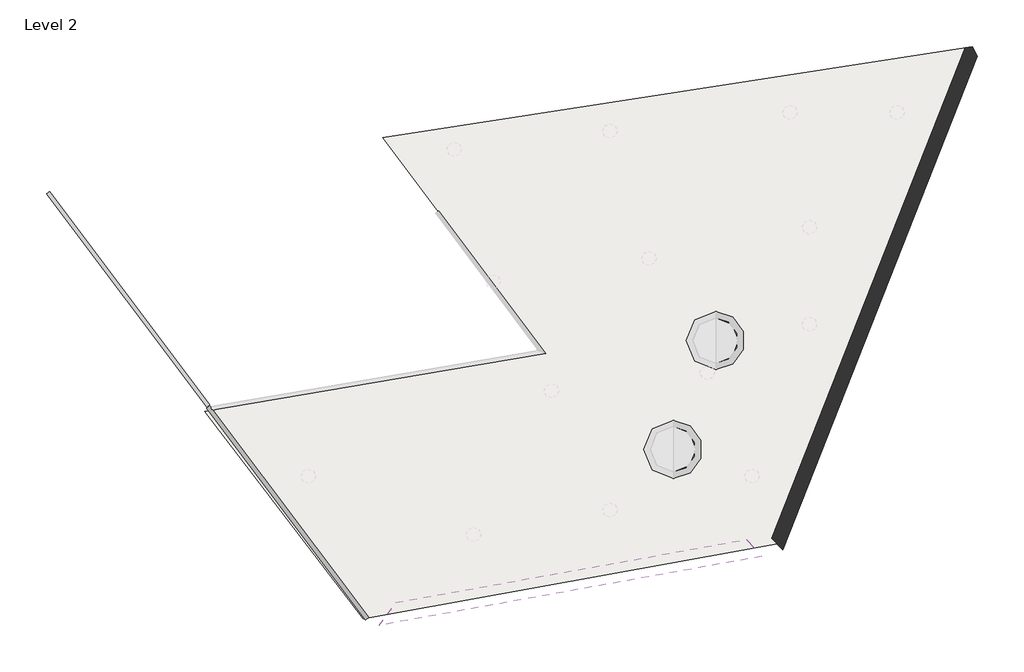
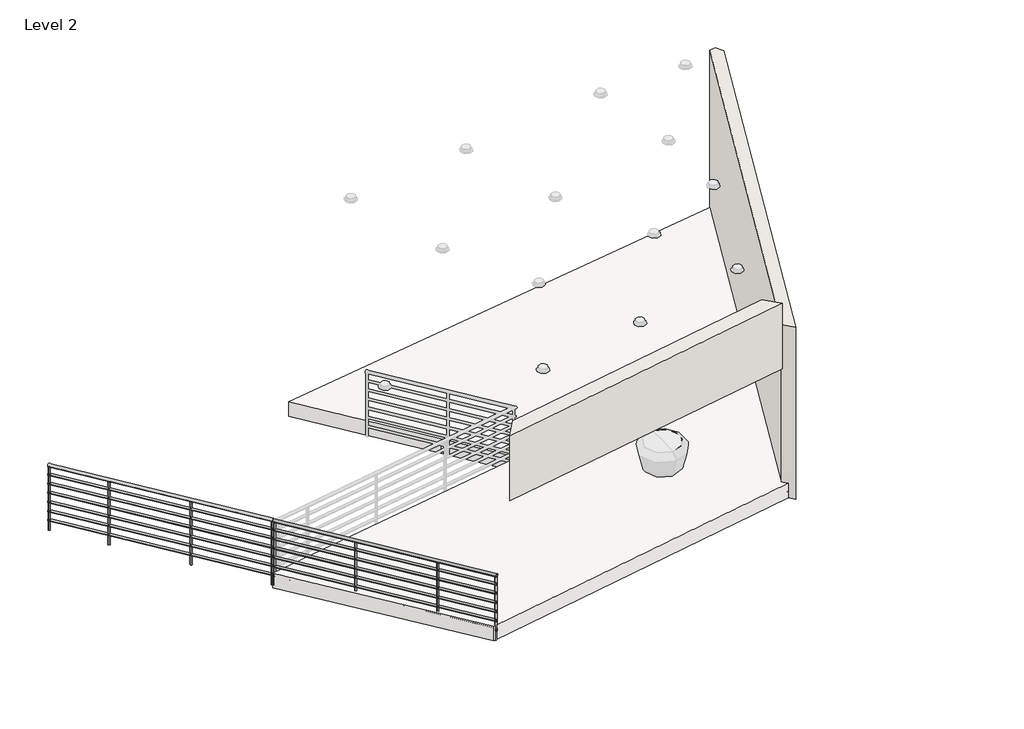
# One storey, part 1 of 2: 2 railings, 2 walls, 1 slab.
"""IFC4 building model written with IfcOpenShell, lengths in millimetres."""

from ifc_helpers import new_model, si_unit, point, frame, frame_2d, origin, place, context, project, spatial, polyline, circle_curve, trimmed, segment, composite_curve, outline, extrude, faceted_brep, element, save
from ifc_brep_helpers import plane_surface, revolved_surface, advanced_brep

model = new_model("IFC4")

# Units and contexts
model_context = context("Model", 3, world=origin())
ifc_project = project(units=[si_unit("LENGTHUNIT", "METRE", prefix="MILLI")], contexts=[model_context])

# Site, building, storey
site = spatial("IfcSite", under=ifc_project)
building = spatial("IfcBuilding", under=site)
storey = spatial("IfcBuildingStorey", under=building, Name="Level 2", Elevation=20000.0)

# Railings
placement = place(None, origin())
element("IfcRailing", 1, ObjectType="900mm Pipe", at=placement, inside=storey, context=model_context, shape_type="SweptSolid", body=[
    extrude(outline(composite_curve([segment(trimmed(circle_curve(frame_2d((0.0, 20.0)), 20.0), [point((-20.0, 20.0))], [point((20.0, 20.0))], False, "CARTESIAN"), True, "CONTINUOUS"), segment(trimmed(circle_curve(frame_2d((0.0, 20.0)), 20.0), [point((20.0, 20.0))], [point((-20.0, 20.0))], False, "CARTESIAN"), True, "CONTINUOUS")], self_intersect=False)), frame((80731.135292, 41327.5386845, 20900.0), z_axis=(-0.600141867985958, 0.7998935793531069, 0.0), x_axis=(0.7998935793531069, 0.600141867985958, 0.0)), (0.0, 0.0, 1.0), 2720.0),
    extrude(outline(composite_curve([segment(trimmed(circle_curve(frame_2d((0.0, 15.0)), 15.0), [point((15.0, 15.0))], [point((-15.0, 15.0))], False, "CARTESIAN"), True, "CONTINUOUS"), segment(trimmed(circle_curve(frame_2d((0.0, 15.0)), 15.0), [point((-15.0, 15.0))], [point((15.0, 15.0))], False, "CARTESIAN"), True, "CONTINUOUS")], self_intersect=False)), frame((80731.135292, 41327.5386845, 20775.0), z_axis=(-0.600141867985958, 0.7998935793531069, 0.0), x_axis=(0.7998935793531069, 0.600141867985958, 0.0)), (0.0, 0.0, 1.0), 2720.0),
    extrude(outline(composite_curve([segment(trimmed(circle_curve(frame_2d((0.0, 15.0)), 15.0), [point((15.0, 15.0))], [point((-15.0, 15.0))], False, "CARTESIAN"), True, "CONTINUOUS"), segment(trimmed(circle_curve(frame_2d((0.0, 15.0)), 15.0), [point((-15.0, 15.0))], [point((15.0, 15.0))], False, "CARTESIAN"), True, "CONTINUOUS")], self_intersect=False)), frame((80731.135292, 41327.5386845, 20650.0), z_axis=(-0.600141867985958, 0.7998935793531069, 0.0), x_axis=(0.7998935793531069, 0.600141867985958, 0.0)), (0.0, 0.0, 1.0), 2720.0),
    extrude(outline(composite_curve([segment(trimmed(circle_curve(frame_2d((0.0, 15.0)), 15.0), [point((15.0, 15.0))], [point((-15.0, 15.0))], False, "CARTESIAN"), True, "CONTINUOUS"), segment(trimmed(circle_curve(frame_2d((0.0, 15.0)), 15.0), [point((-15.0, 15.0))], [point((15.0, 15.0))], False, "CARTESIAN"), True, "CONTINUOUS")], self_intersect=False)), frame((80731.135292, 41327.5386845, 20525.0), z_axis=(-0.600141867985958, 0.7998935793531069, 0.0), x_axis=(0.7998935793531069, 0.600141867985958, 0.0)), (0.0, 0.0, 1.0), 2720.0),
    extrude(outline(composite_curve([segment(trimmed(circle_curve(frame_2d((0.0, 15.0)), 15.0), [point((15.0, 15.0))], [point((-15.0, 15.0))], False, "CARTESIAN"), True, "CONTINUOUS"), segment(trimmed(circle_curve(frame_2d((0.0, 15.0)), 15.0), [point((-15.0, 15.0))], [point((15.0, 15.0))], False, "CARTESIAN"), True, "CONTINUOUS")], self_intersect=False)), frame((80731.135292, 41327.5386845, 20400.0), z_axis=(-0.600141867985958, 0.7998935793531069, 0.0), x_axis=(0.7998935793531069, 0.600141867985958, 0.0)), (0.0, 0.0, 1.0), 2720.0),
    extrude(outline(composite_curve([segment(trimmed(circle_curve(frame_2d((0.0, 15.0)), 15.0), [point((15.0, 15.0))], [point((-15.0, 15.0))], False, "CARTESIAN"), True, "CONTINUOUS"), segment(trimmed(circle_curve(frame_2d((0.0, 15.0)), 15.0), [point((-15.0, 15.0))], [point((15.0, 15.0))], False, "CARTESIAN"), True, "CONTINUOUS")], self_intersect=False)), frame((80731.135292, 41327.5386845, 20275.0), z_axis=(-0.600141867985958, 0.7998935793531069, 0.0), x_axis=(0.7998935793531069, 0.600141867985958, 0.0)), (0.0, 0.0, 1.0), 2720.0),
    extrude(outline(composite_curve([segment(trimmed(circle_curve(frame_2d((0.0, 15.0)), 15.0), [point((15.0, 15.0))], [point((-15.0, 15.0))], False, "CARTESIAN"), True, "CONTINUOUS"), segment(trimmed(circle_curve(frame_2d((0.0, 15.0)), 15.0), [point((-15.0, 15.0))], [point((15.0, 15.0))], False, "CARTESIAN"), True, "CONTINUOUS")], self_intersect=False)), frame((80731.135292, 41327.5386845, 20150.0), z_axis=(-0.600141867985958, 0.7998935793531069, 0.0), x_axis=(0.7998935793531069, 0.600141867985958, 0.0)), (0.0, 0.0, 1.0), 2720.0),
    extrude(outline(composite_curve([segment(trimmed(circle_curve(frame_2d((80299.033147, 41903.4620616)), 12.5), [point((80309.0318168, 41910.963835))], [point((80289.0344773, 41895.9602883))], False, "CARTESIAN"), True, "CONTINUOUS"), segment(trimmed(circle_curve(frame_2d((80299.033147, 41903.4620616)), 12.5), [point((80289.0344773, 41895.9602883))], [point((80309.0318168, 41910.963835))], False, "CARTESIAN"), True, "CONTINUOUS")], self_intersect=False)), frame((0.0, 0.0, 20000.0), z_axis=(0.0, 0.0, 1.0), x_axis=(1.0, 0.0, 0.0)), (0.0, 0.0, 1.0), 860.0),
    extrude(outline(composite_curve([segment(trimmed(circle_curve(frame_2d((79698.8912791, 42703.355641)), 12.5), [point((79708.8899488, 42710.8574143))], [point((79688.8926093, 42695.8538676))], False, "CARTESIAN"), True, "CONTINUOUS"), segment(trimmed(circle_curve(frame_2d((79698.8912791, 42703.355641)), 12.5), [point((79688.8926093, 42695.8538676))], [point((79708.8899488, 42710.8574143))], False, "CARTESIAN"), True, "CONTINUOUS")], self_intersect=False)), frame((0.0, 0.0, 20000.0), z_axis=(0.0, 0.0, 1.0), x_axis=(1.0, 0.0, 0.0)), (0.0, 0.0, 1.0), 860.0),
    extrude(outline(composite_curve([segment(trimmed(circle_curve(frame_2d((80723.6335186, 41337.5373543)), 12.5), [point((80733.6321884, 41345.0391276))], [point((80713.6348489, 41330.0355809))], False, "CARTESIAN"), True, "CONTINUOUS"), segment(trimmed(circle_curve(frame_2d((80723.6335186, 41337.5373543)), 12.5), [point((80713.6348489, 41330.0355809))], [point((80733.6321884, 41345.0391276))], False, "CARTESIAN"), True, "CONTINUOUS")], self_intersect=False)), frame((0.0, 0.0, 20000.0), z_axis=(0.0, 0.0, 1.0), x_axis=(1.0, 0.0, 0.0)), (0.0, 0.0, 1.0), 860.0),
    extrude(outline(composite_curve([segment(trimmed(circle_curve(frame_2d((79106.2511844, 43493.2505506)), 12.5), [point((79116.2498542, 43500.752324))], [point((79096.2525147, 43485.7487773))], False, "CARTESIAN"), True, "CONTINUOUS"), segment(trimmed(circle_curve(frame_2d((79106.2511844, 43493.2505506)), 12.5), [point((79096.2525147, 43485.7487773))], [point((79116.2498542, 43500.752324))], False, "CARTESIAN"), True, "CONTINUOUS")], self_intersect=False)), frame((0.0, 0.0, 20000.0), z_axis=(0.0, 0.0, 1.0), x_axis=(1.0, 0.0, 0.0)), (0.0, 0.0, 1.0), 860.0),
])
element("IfcRailing", 2, ObjectType="900mm Pipe", at=placement, inside=storey, context=model_context, shape_type="SweptSolid", body=[
    extrude(outline(composite_curve([segment(trimmed(circle_curve(frame_2d((0.0, 20.0)), 20.0), [point((20.0, 20.0))], [point((-20.0, 20.0))], False, "CARTESIAN"), True, "CONTINUOUS"), segment(trimmed(circle_curve(frame_2d((0.0, 20.0)), 20.0), [point((-20.0, 20.0))], [point((20.0, 20.0))], False, "CARTESIAN"), True, "CONTINUOUS")], self_intersect=False)), frame((79098.1923254, 43514.614153, 20900.0), z_axis=(-0.6001418679860292, 0.7998935793530534, 0.0), x_axis=(0.7998935793530534, 0.6001418679860292, 0.0)), (0.0, 0.0, 1.0), 2740.0),
    extrude(outline(composite_curve([segment(trimmed(circle_curve(frame_2d((0.0, 15.0)), 15.0), [point((-15.0, 15.0))], [point((15.0000001, 15.0))], False, "CARTESIAN"), True, "CONTINUOUS"), segment(trimmed(circle_curve(frame_2d((0.0, 15.0)), 15.0), [point((15.0000001, 15.0))], [point((-15.0, 15.0))], False, "CARTESIAN"), True, "CONTINUOUS")], self_intersect=False)), frame((79098.1923254, 43514.614153, 20775.0), z_axis=(-0.6001418679860292, 0.7998935793530534, 0.0), x_axis=(0.7998935793530534, 0.6001418679860292, 0.0)), (0.0, 0.0, 1.0), 2740.0),
    extrude(outline(composite_curve([segment(trimmed(circle_curve(frame_2d((0.0, 15.0)), 15.0), [point((-15.0, 15.0))], [point((15.0000001, 15.0))], False, "CARTESIAN"), True, "CONTINUOUS"), segment(trimmed(circle_curve(frame_2d((0.0, 15.0)), 15.0), [point((15.0000001, 15.0))], [point((-15.0, 15.0))], False, "CARTESIAN"), True, "CONTINUOUS")], self_intersect=False)), frame((79098.1923254, 43514.614153, 20650.0), z_axis=(-0.6001418679860292, 0.7998935793530534, 0.0), x_axis=(0.7998935793530534, 0.6001418679860292, 0.0)), (0.0, 0.0, 1.0), 2740.0),
    extrude(outline(composite_curve([segment(trimmed(circle_curve(frame_2d((0.0, 15.0)), 15.0), [point((-15.0, 15.0))], [point((15.0000001, 15.0))], False, "CARTESIAN"), True, "CONTINUOUS"), segment(trimmed(circle_curve(frame_2d((0.0, 15.0)), 15.0), [point((15.0000001, 15.0))], [point((-15.0, 15.0))], False, "CARTESIAN"), True, "CONTINUOUS")], self_intersect=False)), frame((79098.1923254, 43514.614153, 20525.0), z_axis=(-0.6001418679860292, 0.7998935793530534, 0.0), x_axis=(0.7998935793530534, 0.6001418679860292, 0.0)), (0.0, 0.0, 1.0), 2740.0),
    extrude(outline(composite_curve([segment(trimmed(circle_curve(frame_2d((0.0, 15.0)), 15.0), [point((-15.0, 15.0))], [point((15.0000001, 15.0))], False, "CARTESIAN"), True, "CONTINUOUS"), segment(trimmed(circle_curve(frame_2d((0.0, 15.0)), 15.0), [point((15.0000001, 15.0))], [point((-15.0, 15.0))], False, "CARTESIAN"), True, "CONTINUOUS")], self_intersect=False)), frame((79098.1923254, 43514.614153, 20400.0), z_axis=(-0.6001418679860292, 0.7998935793530534, 0.0), x_axis=(0.7998935793530534, 0.6001418679860292, 0.0)), (0.0, 0.0, 1.0), 2740.0),
    extrude(outline(composite_curve([segment(trimmed(circle_curve(frame_2d((0.0, 15.0)), 15.0), [point((-15.0, 15.0))], [point((15.0000001, 15.0))], False, "CARTESIAN"), True, "CONTINUOUS"), segment(trimmed(circle_curve(frame_2d((0.0, 15.0)), 15.0), [point((15.0000001, 15.0))], [point((-15.0, 15.0))], False, "CARTESIAN"), True, "CONTINUOUS")], self_intersect=False)), frame((79098.1923254, 43514.614153, 20275.0), z_axis=(-0.6001418679860292, 0.7998935793530534, 0.0), x_axis=(0.7998935793530534, 0.6001418679860292, 0.0)), (0.0, 0.0, 1.0), 2740.0),
    extrude(outline(composite_curve([segment(trimmed(circle_curve(frame_2d((0.0, 15.0)), 15.0), [point((-15.0, 15.0))], [point((15.0000001, 15.0))], False, "CARTESIAN"), True, "CONTINUOUS"), segment(trimmed(circle_curve(frame_2d((0.0, 15.0)), 15.0), [point((15.0000001, 15.0))], [point((-15.0, 15.0))], False, "CARTESIAN"), True, "CONTINUOUS")], self_intersect=False)), frame((79098.1923254, 43514.614153, 20150.0), z_axis=(-0.6001418679860292, 0.7998935793530534, 0.0), x_axis=(0.7998935793530534, 0.6001418679860292, 0.0)), (0.0, 0.0, 1.0), 2740.0),
    extrude(outline(composite_curve([segment(trimmed(circle_curve(frame_2d((77897.9085894, 45114.4013117)), 12.5), [point((77887.9099197, 45106.8995384))], [point((77907.9072591, 45121.9030851))], False, "CARTESIAN"), True, "CONTINUOUS"), segment(trimmed(circle_curve(frame_2d((77897.9085894, 45114.4013117)), 12.5), [point((77907.9072591, 45121.9030851))], [point((77887.9099197, 45106.8995384))], False, "CARTESIAN"), True, "CONTINUOUS")], self_intersect=False)), frame((0.0, 0.0, 20000.0), z_axis=(0.0, 0.0, 1.0), x_axis=(1.0, 0.0, 0.0)), (0.0, 0.0, 1.0), 860.0),
    extrude(outline(composite_curve([segment(trimmed(circle_curve(frame_2d((78498.0504574, 44314.5077324)), 12.5), [point((78488.0517876, 44307.005959))], [point((78508.0491271, 44322.0095057))], False, "CARTESIAN"), True, "CONTINUOUS"), segment(trimmed(circle_curve(frame_2d((78498.0504574, 44314.5077324)), 12.5), [point((78508.0491271, 44322.0095057))], [point((78488.0517876, 44307.005959))], False, "CARTESIAN"), True, "CONTINUOUS")], self_intersect=False)), frame((0.0, 0.0, 20000.0), z_axis=(0.0, 0.0, 1.0), x_axis=(1.0, 0.0, 0.0)), (0.0, 0.0, 1.0), 860.0),
    extrude(outline(composite_curve([segment(trimmed(circle_curve(frame_2d((77461.3053804, 45696.3238907)), 12.5), [point((77451.3067107, 45688.8221174))], [point((77471.3040502, 45703.8256641))], False, "CARTESIAN"), True, "CONTINUOUS"), segment(trimmed(circle_curve(frame_2d((77461.3053804, 45696.3238907)), 12.5), [point((77471.3040502, 45703.8256641))], [point((77451.3067107, 45688.8221174))], False, "CARTESIAN"), True, "CONTINUOUS")], self_intersect=False)), frame((0.0, 0.0, 20000.0), z_axis=(0.0, 0.0, 1.0), x_axis=(1.0, 0.0, 0.0)), (0.0, 0.0, 1.0), 860.0),
    extrude(outline(composite_curve([segment(trimmed(circle_curve(frame_2d((79090.690552, 43524.6128228)), 12.5), [point((79080.6918823, 43517.1110494))], [point((79100.6892218, 43532.1145961))], False, "CARTESIAN"), True, "CONTINUOUS"), segment(trimmed(circle_curve(frame_2d((79090.690552, 43524.6128228)), 12.5), [point((79100.6892218, 43532.1145961))], [point((79080.6918823, 43517.1110494))], False, "CARTESIAN"), True, "CONTINUOUS")], self_intersect=False)), frame((0.0, 0.0, 20000.0), z_axis=(0.0, 0.0, 1.0), x_axis=(1.0, 0.0, 0.0)), (0.0, 0.0, 1.0), 860.0),
])

# Slab
element("IfcSlab", 3, ObjectType="Generic Floor - 400mm", at=placement, inside=storey, context=model_context, shape_type="AdvancedBrep", body=[
    advanced_brep(
    [(80691.135292, 41327.5386845, 20000.0), (80691.135292, 41327.5386845, 20200.0), (79062.510136, 43459.7811208, 20200.0), (79062.510136, 43459.7811208, 20000.0), (86949.8888821, 47211.4913441, 20200.0), (86949.8888821, 47211.4913441, 20000.0), (80892.7101896, 46274.3130838, 20000.0), (80892.7101896, 46274.3130838, 20200.0), (84946.9218565, 42094.8499105, 20200.0), (84946.9218565, 42094.8499105, 20000.0), (82002.9145503, 44794.5873934, 20200.0), (82567.5701931, 44055.3241449, 20200.0), (82567.5701931, 44055.3241449, 20000.0), (82002.9145503, 44794.5873934, 20000.0), (81497.4034928, 43675.602458, 20000.0), (81387.4034928, 43675.602458, 20000.0), (81045.4161385, 41992.7290245, 20000.0), (80935.4161385, 41992.7290245, 20000.0), (82386.889731, 43815.602458, 20000.0), (82276.889731, 43815.602458, 20000.0), (82225.8855235, 42292.7290245, 20000.0), (82115.8855235, 42292.7290245, 20000.0), (83225.8855235, 42541.7546441, 20000.0), (83115.8855235, 42541.7546441, 20000.0), (82397.6118994, 44592.7290245, 20000.0), (82287.6118994, 44592.7290245, 20000.0), (81506.5966403, 45947.7746156, 20000.0), (81396.5966403, 45947.7746156, 20000.0), (81785.8855235, 42940.1193246, 20000.0), (81675.8855235, 42940.1193246, 20000.0), (80146.889731, 43380.8907492, 20000.0), (80036.889731, 43380.8907492, 20000.0), (80697.4034928, 42375.602458, 20000.0), (80587.4034928, 42375.602458, 20000.0), (81387.4034928, 43675.602458, 20038.1), (81497.4034928, 43675.602458, 20038.1), (80935.4161385, 41992.7290245, 20038.1), (81045.4161385, 41992.7290245, 20038.1), (82276.889731, 43815.602458, 20038.1), (82386.889731, 43815.602458, 20038.1), (82115.8855235, 42292.7290245, 20038.1), (82225.8855235, 42292.7290245, 20038.1), (83115.8855235, 42541.7546441, 20038.1), (83225.8855235, 42541.7546441, 20038.1), (82287.6118994, 44592.7290245, 20038.1), (82397.6118994, 44592.7290245, 20038.1), (81396.5966403, 45947.7746156, 20038.1), (81506.5966403, 45947.7746156, 20038.1), (81675.8855235, 42940.1193246, 20038.1), (81785.8855235, 42940.1193246, 20038.1), (80036.889731, 43380.8907492, 20038.1), (80146.889731, 43380.8907492, 20038.1), (80587.4034928, 42375.602458, 20038.1), (80697.4034928, 42375.602458, 20038.1)],
    [
        (0, 1),
        (1, 2),
        (2, 3),
        (3, 0),
        (4, 5),
        (5, 6),
        (6, 7),
        (7, 4),
        (4, 8),
        (8, 9),
        (9, 5),
        (8, 1),
        (0, 9),
        (7, 10),
        (10, 11),
        (11, 2),
        (3, 12),
        (12, 13),
        (13, 6),
        (14, 15, circle_curve(frame((81442.4034928, 43675.602458, 20000.0), z_axis=(0.0, 0.0, 1.0), x_axis=(1.0, 0.0, 0.0)), 55.0)),
        (15, 14, circle_curve(frame((81442.4034928, 43675.602458, 20000.0), z_axis=(0.0, 0.0, 1.0), x_axis=(1.0, 0.0, 0.0)), 55.0)),
        (16, 17, circle_curve(frame((80990.4161385, 41992.7290245, 20000.0), z_axis=(0.0, 0.0, 1.0), x_axis=(1.0, 0.0, 0.0)), 55.0)),
        (17, 16, circle_curve(frame((80990.4161385, 41992.7290245, 20000.0), z_axis=(0.0, 0.0, 1.0), x_axis=(1.0, 0.0, 0.0)), 55.0)),
        (18, 19, circle_curve(frame((82331.889731, 43815.602458, 20000.0), z_axis=(0.0, 0.0, 1.0), x_axis=(1.0, 0.0, 0.0)), 55.0)),
        (19, 18, circle_curve(frame((82331.889731, 43815.602458, 20000.0), z_axis=(0.0, 0.0, 1.0), x_axis=(1.0, 0.0, 0.0)), 55.0)),
        (20, 21, circle_curve(frame((82170.8855235, 42292.7290245, 20000.0), z_axis=(0.0, 0.0, 1.0), x_axis=(1.0, 0.0, 0.0)), 55.0)),
        (21, 20, circle_curve(frame((82170.8855235, 42292.7290245, 20000.0), z_axis=(0.0, 0.0, 1.0), x_axis=(1.0, 0.0, 0.0)), 55.0)),
        (22, 23, circle_curve(frame((83170.8855235, 42541.7546441, 20000.0), z_axis=(0.0, 0.0, 1.0), x_axis=(1.0, 0.0, 0.0)), 55.0)),
        (23, 22, circle_curve(frame((83170.8855235, 42541.7546441, 20000.0), z_axis=(0.0, 0.0, 1.0), x_axis=(1.0, 0.0, 0.0)), 55.0)),
        (24, 25, circle_curve(frame((82342.6118994, 44592.7290245, 20000.0), z_axis=(0.0, 0.0, 1.0), x_axis=(1.0, 0.0, 0.0)), 55.0)),
        (25, 24, circle_curve(frame((82342.6118994, 44592.7290245, 20000.0), z_axis=(0.0, 0.0, 1.0), x_axis=(1.0, 0.0, 0.0)), 55.0)),
        (26, 27, circle_curve(frame((81451.5966403, 45947.7746156, 20000.0), z_axis=(0.0, 0.0, 1.0), x_axis=(1.0, 0.0, 0.0)), 55.0)),
        (27, 26, circle_curve(frame((81451.5966403, 45947.7746156, 20000.0), z_axis=(0.0, 0.0, 1.0), x_axis=(1.0, 0.0, 0.0)), 55.0)),
        (28, 29, circle_curve(frame((81730.8855235, 42940.1193246, 20000.0), z_axis=(0.0, 0.0, 1.0), x_axis=(1.0, 0.0, 0.0)), 55.0)),
        (29, 28, circle_curve(frame((81730.8855235, 42940.1193246, 20000.0), z_axis=(0.0, 0.0, 1.0), x_axis=(1.0, 0.0, 0.0)), 55.0)),
        (30, 31, circle_curve(frame((80091.889731, 43380.8907492, 20000.0), z_axis=(0.0, 0.0, 1.0), x_axis=(1.0, 0.0, 0.0)), 55.0)),
        (31, 30, circle_curve(frame((80091.889731, 43380.8907492, 20000.0), z_axis=(0.0, 0.0, 1.0), x_axis=(1.0, 0.0, 0.0)), 55.0)),
        (32, 33, circle_curve(frame((80642.4034928, 42375.602458, 20000.0), z_axis=(0.0, 0.0, 1.0), x_axis=(1.0, 0.0, 0.0)), 55.0)),
        (33, 32, circle_curve(frame((80642.4034928, 42375.602458, 20000.0), z_axis=(0.0, 0.0, 1.0), x_axis=(1.0, 0.0, 0.0)), 55.0)),
        (13, 10),
        (11, 12),
        (34, 35, circle_curve(frame((81442.4034928, 43675.602458, 20038.1), z_axis=(0.0, 0.0, -1.0), x_axis=(1.0, 0.0, 0.0)), 55.0)),
        (35, 34, circle_curve(frame((81442.4034928, 43675.602458, 20038.1), z_axis=(0.0, 0.0, -1.0), x_axis=(1.0, 0.0, 0.0)), 55.0)),
        (34, 15),
        (14, 35),
        (36, 37, circle_curve(frame((80990.4161385, 41992.7290245, 20038.1), z_axis=(0.0, 0.0, -1.0), x_axis=(1.0, 0.0, 0.0)), 55.0)),
        (37, 36, circle_curve(frame((80990.4161385, 41992.7290245, 20038.1), z_axis=(0.0, 0.0, -1.0), x_axis=(1.0, 0.0, 0.0)), 55.0)),
        (36, 17),
        (16, 37),
        (38, 39, circle_curve(frame((82331.889731, 43815.602458, 20038.1), z_axis=(0.0, 0.0, -1.0), x_axis=(1.0, 0.0, 0.0)), 55.0)),
        (39, 38, circle_curve(frame((82331.889731, 43815.602458, 20038.1), z_axis=(0.0, 0.0, -1.0), x_axis=(1.0, 0.0, 0.0)), 55.0)),
        (38, 19),
        (18, 39),
        (40, 41, circle_curve(frame((82170.8855235, 42292.7290245, 20038.1), z_axis=(0.0, 0.0, -1.0), x_axis=(1.0, 0.0, 0.0)), 55.0)),
        (41, 40, circle_curve(frame((82170.8855235, 42292.7290245, 20038.1), z_axis=(0.0, 0.0, -1.0), x_axis=(1.0, 0.0, 0.0)), 55.0)),
        (40, 21),
        (20, 41),
        (42, 43, circle_curve(frame((83170.8855235, 42541.7546441, 20038.1), z_axis=(0.0, 0.0, -1.0), x_axis=(1.0, 0.0, 0.0)), 55.0)),
        (43, 42, circle_curve(frame((83170.8855235, 42541.7546441, 20038.1), z_axis=(0.0, 0.0, -1.0), x_axis=(1.0, 0.0, 0.0)), 55.0)),
        (42, 23),
        (22, 43),
        (44, 45, circle_curve(frame((82342.6118994, 44592.7290245, 20038.1), z_axis=(0.0, 0.0, -1.0), x_axis=(1.0, 0.0, 0.0)), 55.0)),
        (45, 44, circle_curve(frame((82342.6118994, 44592.7290245, 20038.1), z_axis=(0.0, 0.0, -1.0), x_axis=(1.0, 0.0, 0.0)), 55.0)),
        (44, 25),
        (24, 45),
        (46, 47, circle_curve(frame((81451.5966403, 45947.7746156, 20038.1), z_axis=(0.0, 0.0, -1.0), x_axis=(1.0, 0.0, 0.0)), 55.0)),
        (47, 46, circle_curve(frame((81451.5966403, 45947.7746156, 20038.1), z_axis=(0.0, 0.0, -1.0), x_axis=(1.0, 0.0, 0.0)), 55.0)),
        (46, 27),
        (26, 47),
        (48, 49, circle_curve(frame((81730.8855235, 42940.1193246, 20038.1), z_axis=(0.0, 0.0, -1.0), x_axis=(1.0, 0.0, 0.0)), 55.0)),
        (49, 48, circle_curve(frame((81730.8855235, 42940.1193246, 20038.1), z_axis=(0.0, 0.0, -1.0), x_axis=(1.0, 0.0, 0.0)), 55.0)),
        (48, 29),
        (28, 49),
        (50, 51, circle_curve(frame((80091.889731, 43380.8907492, 20038.1), z_axis=(0.0, 0.0, -1.0), x_axis=(1.0, 0.0, 0.0)), 55.0)),
        (51, 50, circle_curve(frame((80091.889731, 43380.8907492, 20038.1), z_axis=(0.0, 0.0, -1.0), x_axis=(1.0, 0.0, 0.0)), 55.0)),
        (50, 31),
        (30, 51),
        (52, 53, circle_curve(frame((80642.4034928, 42375.602458, 20038.1), z_axis=(0.0, 0.0, -1.0), x_axis=(1.0, 0.0, 0.0)), 55.0)),
        (53, 52, circle_curve(frame((80642.4034928, 42375.602458, 20038.1), z_axis=(0.0, 0.0, -1.0), x_axis=(1.0, 0.0, 0.0)), 55.0)),
        (52, 33),
        (32, 53),
    ],
    [
        plane_surface(frame((80691.135292, 41327.5386845, 20000.0), z_axis=(-0.7947017778365444, -0.6070000694426944, 0.0), x_axis=(0.0, 0.0, 1.0))),
        plane_surface(frame((80874.8034875, 46271.5425246, 20000.0), z_axis=(-0.1529025770030847, 0.9882412670728823, 0.0), x_axis=(0.0, 0.0, 1.0))),
        plane_surface(frame((86949.8888821, 47211.4913441, 20000.0), z_axis=(0.9311931800132943, -0.36452607793781866, 0.0), x_axis=(0.0, 0.0, 1.0))),
        plane_surface(frame((84946.9218565, 42094.8499105, 20000.0), z_axis=(0.17743737654337016, -0.9841320934739434, 0.0), x_axis=(0.0, 0.0, 1.0))),
        plane_surface(frame((82515.4716412, 44070.0879549, 20200.0), z_axis=(0.0, 0.0, 1.0000000000000002), x_axis=(0.36452607793781866, 0.9311931800132943, 0.0))),
        plane_surface(frame((82515.4716412, 44070.0879549, 20000.0), z_axis=(0.0, 0.0, -1.0000000000000002), x_axis=(0.36452607793781866, 0.9311931800132943, 0.0))),
        plane_surface(frame((82540.2397468, 44078.4184381, 20704.8), z_axis=(-0.7998935793530568, -0.6001418679860248, 0.0), x_axis=(0.0, 0.0, -1.0))),
        plane_surface(frame((79062.510136, 43459.7811208, 20000.0), z_axis=(-0.1675087841932214, 0.9858705834023596, 0.0), x_axis=(0.0, 0.0, 1.0))),
        plane_surface(frame((82567.5701931, 44055.3241449, 20000.0), z_axis=(-0.7947017778365394, -0.6070000694427009, 0.0), x_axis=(0.0, 0.0, 1.0))),
        plane_surface(frame((81497.4034928, 43675.602458, 20038.1), z_axis=(0.0, 0.0, -1.0), x_axis=(0.0, 1.0, 0.0))),
        revolved_surface(polyline([(81497.4034928, 43675.602458, 20000.0), (81497.4034928, 43675.602458, 20038.1)]), (81442.4034928, 43675.602458, 20038.1), (0.0, 0.0, -1.0)),
        plane_surface(frame((81045.4161385, 41992.7290245, 20038.1), z_axis=(0.0, 0.0, -1.0), x_axis=(0.0, 1.0, 0.0))),
        revolved_surface(polyline([(81045.4161385, 41992.7290245, 20000.0), (81045.4161385, 41992.7290245, 20038.1)]), (80990.4161385, 41992.7290245, 20038.1), (0.0, 0.0, -1.0)),
        plane_surface(frame((82386.889731, 43815.602458, 20038.1), z_axis=(0.0, 0.0, -1.0), x_axis=(0.0, 1.0, 0.0))),
        revolved_surface(polyline([(82386.889731, 43815.602458, 20000.0), (82386.889731, 43815.602458, 20038.1)]), (82331.889731, 43815.602458, 20038.1), (0.0, 0.0, -1.0)),
        plane_surface(frame((82225.8855235, 42292.7290245, 20038.1), z_axis=(0.0, 0.0, -1.0), x_axis=(0.0, 1.0, 0.0))),
        revolved_surface(polyline([(82225.8855235, 42292.7290245, 20000.0), (82225.8855235, 42292.7290245, 20038.1)]), (82170.8855235, 42292.7290245, 20038.1), (0.0, 0.0, -1.0)),
        plane_surface(frame((83225.8855235, 42541.7546441, 20038.1), z_axis=(0.0, 0.0, -1.0), x_axis=(0.0, 1.0, 0.0))),
        revolved_surface(polyline([(83225.8855235, 42541.7546441, 20000.0), (83225.8855235, 42541.7546441, 20038.1)]), (83170.8855235, 42541.7546441, 20038.1), (0.0, 0.0, -1.0)),
        plane_surface(frame((82397.6118994, 44592.7290245, 20038.1), z_axis=(0.0, 0.0, -1.0), x_axis=(0.0, 1.0, 0.0))),
        revolved_surface(polyline([(82397.6118994, 44592.7290245, 20000.0), (82397.6118994, 44592.7290245, 20038.1)]), (82342.6118994, 44592.7290245, 20038.1), (0.0, 0.0, -1.0)),
        plane_surface(frame((81506.5966403, 45947.7746156, 20038.1), z_axis=(0.0, 0.0, -1.0), x_axis=(0.0, 1.0, 0.0))),
        revolved_surface(polyline([(81506.5966403, 45947.7746156, 20000.0), (81506.5966403, 45947.7746156, 20038.1)]), (81451.5966403, 45947.7746156, 20038.1), (0.0, 0.0, -1.0)),
        plane_surface(frame((81785.8855235, 42940.1193246, 20038.1), z_axis=(0.0, 0.0, -1.0), x_axis=(0.0, 1.0, 0.0))),
        revolved_surface(polyline([(81785.8855235, 42940.1193246, 20000.0), (81785.8855235, 42940.1193246, 20038.1)]), (81730.8855235, 42940.1193246, 20038.1), (0.0, 0.0, -1.0)),
        plane_surface(frame((80146.889731, 43380.8907492, 20038.1), z_axis=(0.0, 0.0, -1.0), x_axis=(0.0, 1.0, 0.0))),
        revolved_surface(polyline([(80146.889731, 43380.8907492, 20000.0), (80146.889731, 43380.8907492, 20038.1)]), (80091.889731, 43380.8907492, 20038.1), (0.0, 0.0, -1.0)),
        plane_surface(frame((80697.4034928, 42375.602458, 20038.1), z_axis=(0.0, 0.0, -1.0), x_axis=(0.0, 1.0, 0.0))),
        revolved_surface(polyline([(80697.4034928, 42375.602458, 20000.0), (80697.4034928, 42375.602458, 20038.1)]), (80642.4034928, 42375.602458, 20038.1), (0.0, 0.0, -1.0)),
    ],
    [
        (0, [[1, 2, 3, 4]]),
        (1, [[5, 6, 7, 8]]),
        (2, [[-5, 9, 10, 11]]),
        (3, [[-10, 12, -1, 13]]),
        (4, [[-12, -9, -8, 14, 15, 16, -2]]),
        (5, [[-11, -13, -4, 17, 18, 19, -6], [20, 21], [22, 23], [24, 25], [26, 27], [28, 29], [30, 31], [32, 33], [34, 35], [36, 37], [38, 39]]),
        (6, [[-7, -19, 40, -14]]),
        (7, [[-3, -16, 41, -17]]),
        (8, [[-41, -15, -40, -18]]),
        (9, [[42, 43]]),
        (10, [[-42, 44, -20, 45]]),
        (10, [[-43, -45, -21, -44]]),
        (11, [[46, 47]]),
        (12, [[-46, 48, -22, 49]]),
        (12, [[-47, -49, -23, -48]]),
        (13, [[50, 51]]),
        (14, [[-50, 52, -24, 53]]),
        (14, [[-51, -53, -25, -52]]),
        (15, [[54, 55]]),
        (16, [[-54, 56, -26, 57]]),
        (16, [[-55, -57, -27, -56]]),
        (17, [[58, 59]]),
        (18, [[-58, 60, -28, 61]]),
        (18, [[-59, -61, -29, -60]]),
        (19, [[62, 63]]),
        (20, [[-62, 64, -30, 65]]),
        (20, [[-63, -65, -31, -64]]),
        (21, [[66, 67]]),
        (22, [[-66, 68, -32, 69]]),
        (22, [[-67, -69, -33, -68]]),
        (23, [[70, 71]]),
        (24, [[-70, 72, -34, 73]]),
        (24, [[-71, -73, -35, -72]]),
        (25, [[74, 75]]),
        (26, [[-74, 76, -36, 77]]),
        (26, [[-75, -77, -37, -76]]),
        (27, [[78, 79]]),
        (28, [[-78, 80, -38, 81]]),
        (28, [[-79, -81, -39, -80]]),
    ],
),
])

# Walls
element("IfcWall", 4, ObjectType="Generic - 150mm", at=placement, inside=storey, context=model_context, shape_type="Brep", body=[
    faceted_brep([(86878.6302202, 47200.4660678, 20000.0), (84861.6234348, 42082.2312827, 20000.0), (84861.6234348, 42082.2312827, 20091.1508296), (84890.0021127, 42154.2433046, 20091.1508296), (84890.0021127, 42154.2433046, 22350.0), (86878.6302202, 47200.4660678, 22350.0), (87005.5516332, 47113.4132762, 20000.0), (87005.5516332, 47113.4132762, 22350.0), (85003.3348817, 42032.7087893, 22350.0), (85003.3348817, 42032.7087893, 20000.0), (86952.4470552, 47211.8871495, 20000.0), (86999.2984451, 47125.0088048, 20000.0), (84943.4044863, 42096.9762701, 20000.0), (86952.4470552, 47211.8871495, 22350.0), (84943.4044863, 42096.9762701, 20091.1508296)], [[[0, 1, 2, 3, 4, 5]], [[6, 7, 8, 9]], [[1, 0, 10, 11, 6, 9, 12]], [[5, 4, 8, 7, 13]], [[0, 5, 13, 10]], [[13, 7, 6, 11, 10]], [[2, 1, 12, 14]], [[14, 3, 2]], [[3, 14, 12, 9, 8, 4]]]),
])
element("IfcWall", 5, ObjectType="Generic - 200mm", at=placement, inside=storey, context=model_context, shape_type="Brep", body=[
    faceted_brep([(84628.1824848, 42141.7546441, 22790.0), (84628.1824848, 42141.7546441, 21895.4), (81028.4508259, 41492.7290245, 21895.4), (81028.4508259, 41492.7290245, 22790.0), (84790.4161385, 41967.7803502, 21895.4), (84790.4161385, 41967.7803502, 22790.0), (80856.3561598, 41258.4758916, 22790.0), (80856.3561598, 41258.4758916, 21895.4), (84709.2993116, 42054.7674972, 21895.4), (80942.4034928, 41375.602458, 21895.4)], [[[0, 1, 2, 3]], [[4, 5, 6, 7]], [[2, 1, 8, 4, 7, 9]], [[0, 3, 6, 5]], [[3, 2, 9, 7, 6]], [[0, 5, 4, 8, 1]]]),
])

save(model, "model.ifc")

# Revit data of these elements
# Project information
#   Project Issue Date = "05/22/2020"
#   Project Status = "Project  Status"
#   Project Address = "## Street\nCity, State  Zip"
#   Project Number = "1"
# Type "900mm Pipe"
#   built-in parameter 1008612 = 0.019685 (stored number, unit not read)
#   built-in parameter 1008611 = 0.0984252 (stored number, unit not read)
#   built-in parameter 1008609 = 6.56168 (stored number, unit not read)
#   built-in parameter 1008604 = 0.19685 (stored number, unit not read)
#   built-in parameter 1008603 = 0.164042 (stored number, unit not read)
#   Railing Height = 0.9 m
#   built-in parameter 1008630 = 2
#   built-in parameter 1008610 = 2
#   built-in parameter 1008605 = 1
#   built-in parameter 1008618 = M_Baluster - Round : 25mm
# Type "Generic Floor - 400mm"
#   Function = 0
#   Layers, outside or top first: 0.2 m "Wood - Birch - Solid Stained Light Low Gloss" (function 1)
# Type "Generic - 150mm"
#   Layers, outside or top first: 0.15 m "Concrete, Lightweight" (function 1)
# Type "Generic - 200mm"
#   Layers, outside or top first: 0.2 m "Concrete, Lightweight" (function 1)
# Elements 1, 2 (IfcRailing, "900mm Pipe")
#   Phase Created = New Construction
# Element 3 (IfcSlab, "Generic Floor - 400mm")
#   built-in parameter 1001955 = -0.918516 (stored number, unit not read)
#   Height Offset From Level = 0.2 m
#   Phase Created = New Construction
#   Materials on its faces: "Wood - Birch - Solid Stained Light Low Gloss"
# Element 4 (IfcWall, "Generic - 150mm")
#   Top Offset = 0 m
#   Base Offset = 0 m
#   Unconnected Height = 2.35 m
#   wall height = 2.35 m
#   Phase Created = New Construction
#   Base Constraint = Level 2
#   Materials on its faces: "Concrete, Lightweight"
# Element 5 (IfcWall, "Generic - 200mm")
#   built-in parameter 1001111 = 1.8954 m
#   Top Offset = 0 m
#   Base Offset = 1.8954 m
#   Unconnected Height = 0.8946 m
#   wall height = 0.8946 m
#   Phase Created = New Construction
#   Base Constraint = Level 2
#   Materials on its faces: "Concrete, Lightweight"
# Materials
#   "Wood - Birch - Solid Stained Light Low Gloss": class "Wood", colour RGB 227 170 128, transparency 0, Cost = 0
#   "Concrete, Lightweight": class "Concrete", colour RGB 129 132 118, transparency 0, Description = "Lightweight concrete", Cost = 0
